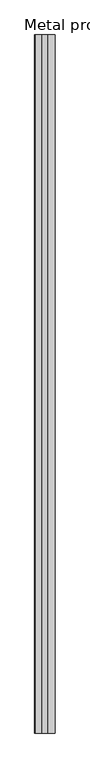
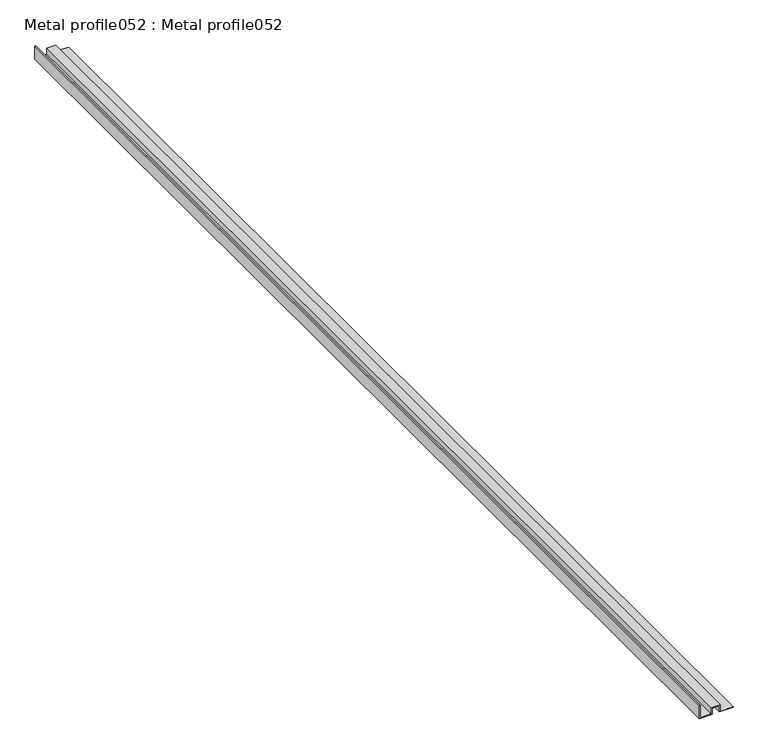
"""IFC4 building model written with IfcOpenShell, lengths in millimetres: proxy geometry, Metal profile052 : Metal profile052."""

from ifc_helpers import new_model, si_unit, frame, origin, place, context, project, spatial, polyline, outline, extrude, source, transform, mapped, element, save


def metal_profile052_metal_profile052_f9a601b4(model_context):
    return source(origin(), model_context, "Body", "SweptSolid", [
        extrude(outline(polyline([(39543.8875708, -5021.2557575), (39543.8875708, -4999.0307575), (39555.3175708, -4999.0307575), (39555.3175708, -4986.3307575), (39543.8875708, -4986.3307575), (39543.8875708, -4962.6175735), (39545.1675708, -4962.6175735), (39545.1675708, -4985.0507575), (39556.5975708, -4985.0507575), (39556.5975708, -5000.3107575), (39545.1675708, -5000.3107575), (39545.1675708, -5019.9757575), (39567.6883323, -5019.9757575), (39567.6883323, -5021.2557575), (39543.8875708, -5021.2557575)])), frame((0.0, -1052.8906574, 0.0), z_axis=(0.0, 1.0, 0.0), x_axis=(0.0, 0.0, 1.0)), (0.0, 0.0, 1.0), 2000.0),
    ])


if __name__ == "__main__":
    model = new_model("IFC4")
    model_context = context("Model", 3, world=origin())
    ifc_project = project(units=[si_unit("LENGTHUNIT", "METRE", prefix="MILLI")], contexts=[model_context])
    site = spatial("IfcSite", under=ifc_project)
    building = spatial("IfcBuilding", under=site)
    placement = place(None, origin())
    metal_profile052_metal_profile052_shape = metal_profile052_metal_profile052_f9a601b4(model_context)
    element("IfcBuildingElementProxy", 1, Name="Metal profile052 : Metal profile052", ObjectType="Metal profile052 : Metal profile052", at=placement, inside=building, context=model_context, shape_type="MappedRepresentation", body=[
        mapped(metal_profile052_metal_profile052_shape, transform((0.0, 0.0, 0.0), x_axis=(1.0, 0.0, 0.0), y_axis=(0.0, 1.0, 0.0), z_axis=(0.0, 0.0, 1.0))),
    ])
    save(model, "model.ifc")

# Revit data of these elements
# Type "Metal profile052 : Metal profile052"
#   NameOverride = "Metal profile052"
# Element 1 (IfcBuildingElementProxy, "Metal profile052 : Metal profile052")
#   Materials on its faces: "16 GA. COPPER SOFFIT DRIP SCREED"
# Materials
#   "16 GA. COPPER SOFFIT DRIP SCREED": class "Unassigned", colour RGB 255 217 0, transparency 0
